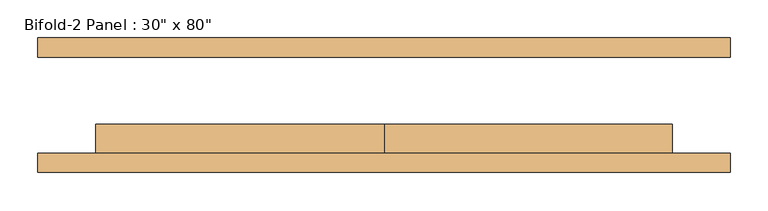
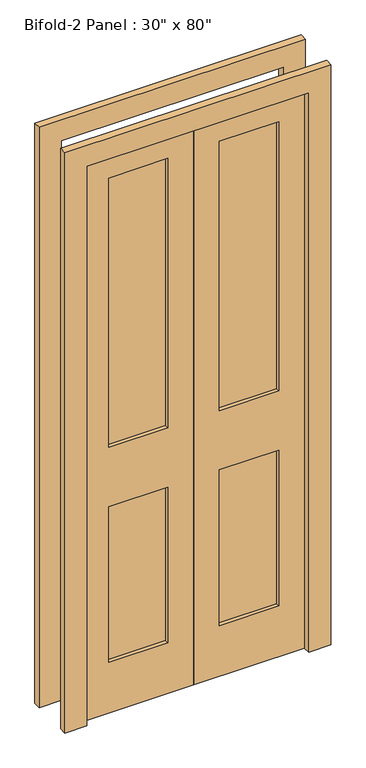
"""IFC4 building model written with IfcOpenShell, lengths in millimetres: door geometry."""

import ifcopenshell
import ifcopenshell.guid

model = None  # the IFC model being written
_history = None  # IfcOwnerHistory: only IFC2X3 demands one
_inside = {}  # id of a spatial element -> (the spatial element, [elements in it])
_under = {}  # id of a project, library or spatial element -> (it, [spatial elements below it])
_declared = {}  # id of a project -> (the project, [libraries it declares])
_typed = {}  # id of a type object -> (the type object, [elements of that type])
_made_of = {}  # id of a material, layer set ... -> (it, [elements and type objects made of it])


def new_model(schema):
    """Start an empty IFC model of exactly this schema.

    Asked for "IFC4X3", IfcOpenShell would pick the latest addendum, in which some entities
    have other attributes; the version numbers below select the first issue.
    IFC2X3 requires an IfcOwnerHistory on every rooted entity: one is made here for all.
    """
    global model, _history
    if schema == "IFC4X3":
        model = ifcopenshell.file(schema_version=(4, 3, 0, 0))
    else:
        model = ifcopenshell.file(schema=schema)
    _inside.clear()
    _under.clear()
    _declared.clear()
    _typed.clear()
    _made_of.clear()
    _history = None
    if model.schema == "IFC2X3":
        org = make("IfcOrganization", Name="unknown")
        user = make(
            "IfcPersonAndOrganization",
            ThePerson=make("IfcPerson", FamilyName="unknown"),
            TheOrganization=org,
        )
        app = make(
            "IfcApplication",
            ApplicationDeveloper=org,
            Version="unknown",
            ApplicationFullName="unknown",
            ApplicationIdentifier="unknown",
        )
        _history = make(
            "IfcOwnerHistory",
            OwningUser=user,
            OwningApplication=app,
            ChangeAction="ADDED",
            CreationDate=0,
        )
    return model


def make(cls, **values):
    """One entity of the class cls with the attributes given. An attribute that is None is left unset."""
    return model.create_entity(
        cls, **{name: value for name, value in values.items() if value is not None}
    )


def rooted(cls, **values):
    """An entity with a GlobalId (a new one), such as an element, a storey or a relation."""
    return make(cls, GlobalId=ifcopenshell.guid.new(), OwnerHistory=_history, **values)


def si_unit(unit_type, name, prefix=None):
    """IfcSIUnit, for example si_unit("LENGTHUNIT", "METRE", prefix="MILLI")."""
    return make("IfcSIUnit", UnitType=unit_type, Prefix=prefix, Name=name)


def assignment(units):
    """IfcUnitAssignment: the units of a project."""
    return None if units is None else make("IfcUnitAssignment", Units=units)


def point(xyz):
    """IfcCartesianPoint."""
    return None if xyz is None else make("IfcCartesianPoint", Coordinates=xyz)


def direction(xyz):
    """IfcDirection."""
    return None if xyz is None else make("IfcDirection", DirectionRatios=xyz)


def frame(location, z_axis=None, x_axis=None):
    """IfcAxis2Placement3D, a coordinate frame: its origin and axes. An axis left out is left unset."""
    return make(
        "IfcAxis2Placement3D",
        Location=point(location),
        Axis=direction(z_axis),
        RefDirection=direction(x_axis),
    )


def origin():
    """The frame at (0, 0, 0) with its axes left unset."""
    return frame((0.0, 0.0, 0.0))


def place(relative_to, where):
    """IfcLocalPlacement: puts the frame where relative to a parent placement (None: the world)."""
    return make(
        "IfcLocalPlacement", PlacementRelTo=relative_to, RelativePlacement=where
    )


def context(
    kind, dimensions, precision=None, world=None, true_north=None, identifier=None
):
    """IfcGeometricRepresentationContext, for example the 3D "Model" context."""
    return make(
        "IfcGeometricRepresentationContext",
        ContextIdentifier=identifier,
        ContextType=kind,
        CoordinateSpaceDimension=dimensions,
        Precision=precision,
        WorldCoordinateSystem=world,
        TrueNorth=true_north,
    )


def project(units=None, contexts=None):
    """IfcProject with its units and contexts."""
    return rooted(
        "IfcProject",
        Name="project",
        RepresentationContexts=contexts,
        UnitsInContext=assignment(units),
    )


def spatial(cls, under=None, at=None, **own):
    """A site, building, storey or space (cls), placed at a placement, below another one or the project."""
    s = rooted(cls, ObjectPlacement=at, **own)
    if under is not None:
        _under.setdefault(under.id(), (under, []))[1].append(s)
    return s


def polyline(points):
    """IfcPolyline through the points."""
    return make("IfcPolyline", Points=[point(p) for p in points])


def outline(outer, holes=None, kind="AREA"):
    """IfcArbitraryClosedProfileDef: a profile drawn as a closed curve; with holes, ...WithVoids."""
    if holes is None:
        return make("IfcArbitraryClosedProfileDef", ProfileType=kind, OuterCurve=outer)
    return make(
        "IfcArbitraryProfileDefWithVoids",
        ProfileType=kind,
        OuterCurve=outer,
        InnerCurves=holes,
    )


def extrude(swept, where, along, depth):
    """IfcExtrudedAreaSolid: the profile swept, set in the frame where, extruded along a direction by depth."""
    return make(
        "IfcExtrudedAreaSolid",
        SweptArea=swept,
        Position=where,
        ExtrudedDirection=direction(along),
        Depth=depth,
    )


def shape(context_of_items, identifier, shape_type, items):
    """IfcShapeRepresentation: the items that make up one representation, for example the "Body"."""
    return make(
        "IfcShapeRepresentation",
        ContextOfItems=context_of_items,
        RepresentationIdentifier=identifier,
        RepresentationType=shape_type,
        Items=items,
    )


def source(mapping_origin, context_of_items, identifier, shape_type, items):
    """IfcRepresentationMap: a shape defined once, which mapped items show again and again."""
    return make(
        "IfcRepresentationMap",
        MappingOrigin=mapping_origin,
        MappedRepresentation=shape(context_of_items, identifier, shape_type, items),
    )


def transform(
    local_origin,
    x_axis=None,
    y_axis=None,
    z_axis=None,
    scale=None,
    scale2=None,
    scale3=None,
    uniform=True,
):
    """IfcCartesianTransformationOperator3D, or its non-uniform kind. x_axis, y_axis, z_axis: its Axis1, 2, 3."""
    if uniform:
        return make(
            "IfcCartesianTransformationOperator3D",
            Axis1=direction(x_axis),
            Axis2=direction(y_axis),
            LocalOrigin=point(local_origin),
            Scale=scale,
            Axis3=direction(z_axis),
        )
    return make(
        "IfcCartesianTransformationOperator3DnonUniform",
        Axis1=direction(x_axis),
        Axis2=direction(y_axis),
        LocalOrigin=point(local_origin),
        Scale=scale,
        Axis3=direction(z_axis),
        Scale2=scale2,
        Scale3=scale3,
    )


def mapped(mapping_source, mapping_target):
    """IfcMappedItem: shows the shape of a source again, moved by a transform."""
    return make(
        "IfcMappedItem", MappingSource=mapping_source, MappingTarget=mapping_target
    )


def made_of(thing, what):
    """Note that an element or type object is made of a material, layer set ...; save() writes the relation."""
    if what is not None:
        _made_of.setdefault(what.id(), (what, []))[1].append(thing)
    return thing


def element(
    cls,
    number,
    at=None,
    inside=None,
    cuts=None,
    type_object=None,
    material=None,
    context=None,
    identifier="Body",
    shape_type=None,
    held_by="IfcProductDefinitionShape",
    body=None,
    shapes=None,
    **own,
):
    """One element of the class cls, such as IfcWall. Its Tag is "e" and its number.

    at: its placement. inside: the storey or other place that contains it. cuts: it is an
    opening in that element (IfcRelVoidsElement). A single representation is given by context,
    identifier, shape_type and body (its items); several are given by shapes. held_by: the class
    of the entity that holds the representations. save() writes the other relations.
    """
    e = rooted(cls, Tag="e%d" % number, ObjectPlacement=at, **own)
    if body is not None:
        shapes = [shape(context, identifier, shape_type, body)]
    if shapes is not None:
        e.Representation = make(held_by, Representations=shapes)
    if inside is not None:
        _inside.setdefault(inside.id(), (inside, []))[1].append(e)
    if cuts is not None:
        rooted(
            "IfcRelVoidsElement", RelatingBuildingElement=cuts, RelatedOpeningElement=e
        )
    if type_object is not None:
        _typed.setdefault(type_object.id(), (type_object, []))[1].append(e)
    return made_of(e, material)


def aggregate(whole, parts):
    """IfcRelAggregates: a whole, such as a stair, and the parts it consists of."""
    return rooted("IfcRelAggregates", RelatingObject=whole, RelatedObjects=parts)


def save(model, path):
    """Write the relations noted so far, then the file.

    IfcRelAggregates (storeys below a building ...), IfcRelContainedInSpatialStructure (elements
    in a storey), IfcRelDefinesByType, IfcRelAssociatesMaterial and IfcRelDeclares: one each for
    every whole, place, type object, material and project.
    """
    for whole, parts in _under.values():
        aggregate(whole, parts)
    for where, things in _inside.values():
        rooted(
            "IfcRelContainedInSpatialStructure",
            RelatedElements=things,
            RelatingStructure=where,
        )
    for kind, things in _typed.values():
        rooted("IfcRelDefinesByType", RelatedObjects=things, RelatingType=kind)
    for what, things in _made_of.values():
        rooted("IfcRelAssociatesMaterial", RelatedObjects=things, RelatingMaterial=what)
    for by, libraries in _declared.values():
        rooted("IfcRelDeclares", RelatingContext=by, RelatedDefinitions=libraries)
    model.write(path)


def door_22ba5e7f(model_context):
    return source(origin(), model_context, "Body", "SweptSolid", [
        extrude(outline(polyline([(2032.0, 0.0), (2032.0, -381.0), (0.0, -381.0), (0.0, 0.0), (2032.0, 0.0)]), holes=[polyline([(1943.1, -88.9), (965.11872, -88.9), (965.11872, -292.1), (1943.1, -292.1), (1943.1, -88.9)]), polyline([(749.3, -88.9), (184.15, -88.9), (184.15, -292.1), (749.3, -292.1), (749.3, -88.9)])]), frame((0.0, -63.5, 0.0), z_axis=(0.0, 1.0, 0.0), x_axis=(0.0, 0.0, 1.0)), (0.0, 0.0, 1.0), 38.1),
        extrude(outline(polyline([(-88.9, -38.1), (-88.9, -50.8), (-292.1, -50.8), (-292.1, -38.1), (-88.9, -38.1)])), frame((0.0, 0.0, 965.11872), z_axis=(0.0, 0.0, 1.0), x_axis=(1.0, 0.0, 0.0)), (0.0, 0.0, 1.0), 977.98128),
        extrude(outline(polyline([(-88.9, -38.1), (-88.9, -50.8), (-292.1, -50.8), (-292.1, -38.1), (-88.9, -38.1)])), frame((0.0, 0.0, 184.15), z_axis=(0.0, 0.0, 1.0), x_axis=(1.0, 0.0, 0.0)), (0.0, 0.0, 1.0), 565.15),
        extrude(outline(polyline([(292.1, -38.1), (292.1, -50.8), (88.9, -50.8), (88.9, -38.1), (292.1, -38.1)])), frame((0.0, 0.0, 965.11872), z_axis=(0.0, 0.0, 1.0), x_axis=(1.0, 0.0, 0.0)), (0.0, 0.0, 1.0), 977.98128),
        extrude(outline(polyline([(292.1, -38.1), (292.1, -50.8), (88.9, -50.8), (88.9, -38.1), (292.1, -38.1)])), frame((0.0, 0.0, 184.15), z_axis=(0.0, 0.0, 1.0), x_axis=(1.0, 0.0, 0.0)), (0.0, 0.0, 1.0), 565.15),
        extrude(outline(polyline([(2108.2, -457.2), (0.0, -457.2), (0.0, -381.0), (2032.0, -381.0), (2032.0, 381.0), (0.0, 381.0), (0.0, 457.2), (2108.2, 457.2), (2108.2, -457.2)])), frame((0.0, -88.9, 0.0), z_axis=(0.0, 1.0, 0.0), x_axis=(0.0, 0.0, 1.0)), (0.0, 0.0, 1.0), 25.4),
        extrude(outline(polyline([(2108.2, 457.2), (2108.2, -457.2), (0.0, -457.2), (0.0, -381.0), (2032.0, -381.0), (2032.0, 381.0), (0.0, 381.0), (0.0, 457.2), (2108.2, 457.2)])), frame((0.0, 63.5, 0.0), z_axis=(0.0, 1.0, 0.0), x_axis=(0.0, 0.0, 1.0)), (0.0, 0.0, 1.0), 25.4),
        extrude(outline(polyline([(2032.0, 381.0), (2032.0, 0.0), (0.0, 0.0), (0.0, 381.0), (2032.0, 381.0)]), holes=[polyline([(1943.1, 88.9), (1943.1, 292.1), (965.11872, 292.1), (965.11872, 88.9), (1943.1, 88.9)]), polyline([(749.3, 88.9), (749.3, 292.1), (184.15, 292.1), (184.15, 88.9), (749.3, 88.9)])]), frame((0.0, -63.5, 0.0), z_axis=(0.0, 1.0, 0.0), x_axis=(0.0, 0.0, 1.0)), (0.0, 0.0, 1.0), 38.1),
    ])


if __name__ == "__main__":
    model = new_model("IFC4")
    model_context = context("Model", 3, world=origin())
    ifc_project = project(units=[si_unit("LENGTHUNIT", "METRE", prefix="MILLI")], contexts=[model_context])
    site = spatial("IfcSite", under=ifc_project)
    building = spatial("IfcBuilding", under=site)
    placement = place(None, origin())
    door_shape = door_22ba5e7f(model_context)
    element("IfcDoor", 1, ObjectType="Bifold-2 Panel : 30\" x 80\"", at=placement, inside=building, context=model_context, shape_type="MappedRepresentation", body=[
        mapped(door_shape, transform((0.0, 0.0, 0.0), x_axis=(1.0, 0.0, 0.0), y_axis=(0.0, 1.0, 0.0), z_axis=(0.0, 0.0, 1.0))),
    ])
    save(model, "model.ifc")

# Revit data of these elements
# Type "Bifold-2 Panel : 30\" x 80\""
#   Type Mark = "11"
#   Construction Type Id = "MDOOR"
#   Assembly Code = "C1020"
#   Analytic Construction = "Metal"
#   Thickness = 0' - 1 1/2"
#   Thermal Resistance (R) = 1.5338 (h·ft²·°F)/BTU
#   Heat Transfer Coefficient (U) = 0.651978 BTU/(h·ft²·°F)
#   Height = 6' - 8"
#   Trim Projection Ext = 0' - 1"
#   Trim Projection Int = 0' - 1"
#   Trim Width = 0' - 3"
#   Width = 2' - 6"
#   Define Thermal Properties by = 1
#   Door Material = Door - Panel
#   Frame Material = Door - Frame
#   Visual Light Transmittance = 0
#   Solar Heat Gain Coefficient = 0
#   Function = (empty or 0)
#   Wall Closure = (empty or 0)
# Element 1 (IfcDoor, "Bifold-2 Panel : 30\" x 80\"")
#   Materials on its faces: "Door - Panel", "Door - Frame"
# Materials
#   "Door - Panel": class "Wood", colour RGB 210 159 95, transparency 0, Cost = 0
#   "Door - Frame": class "Miscellaneous", colour RGB 118 70 51, transparency 0, Cost = 0
